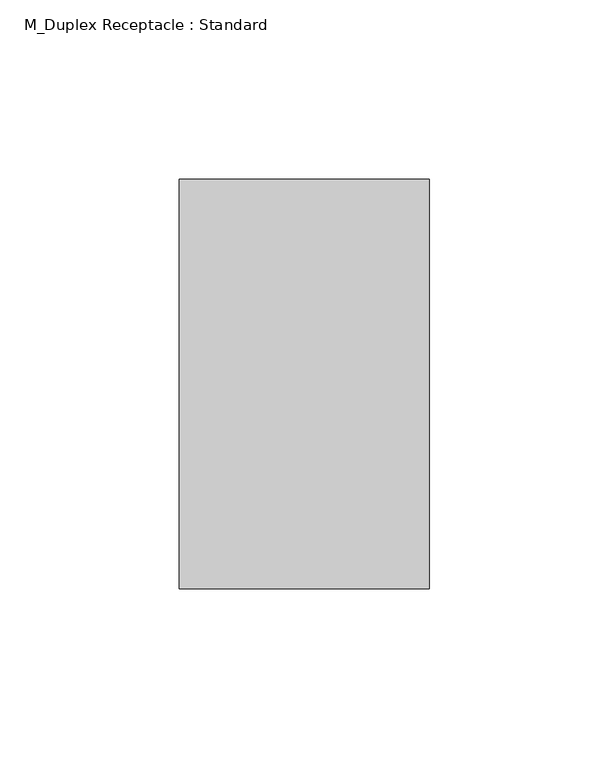
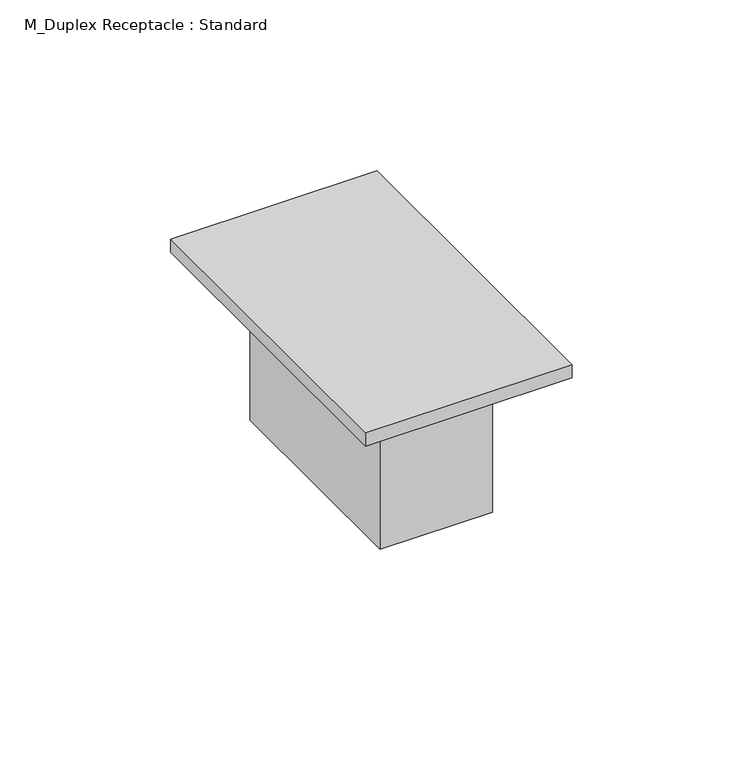
"""IFC4 building model written with IfcOpenShell, lengths in millimetres: proxy geometry, M_Duplex Receptacle : Standard."""

from ifc_helpers import new_model, si_unit, frame, origin, origin_with_axes, place, context, project, spatial, polyline, outline, extrude, source, transform, mapped, element, save


def m_duplex_receptacle_standard_10251bba(model_context):
    return source(origin(), model_context, "Body", "SweptSolid", [
        extrude(outline(polyline([(19.05, 38.1), (19.05, -38.1), (-19.05, -38.1), (-19.05, 38.1), (19.05, 38.1)])), frame((0.0, 0.0, -53.975), z_axis=(0.0, 0.0, 1.0), x_axis=(1.0, 0.0, 0.0)), (0.0, 0.0, 1.0), 53.975),
        extrude(outline(polyline([(34.925, 57.15), (34.925, -57.15), (-34.925, -57.15), (-34.925, 57.15), (34.925, 57.15)])), origin_with_axes(), (0.0, 0.0, 1.0), 4.7625),
    ])


if __name__ == "__main__":
    model = new_model("IFC4")
    model_context = context("Model", 3, world=origin())
    ifc_project = project(units=[si_unit("LENGTHUNIT", "METRE", prefix="MILLI")], contexts=[model_context])
    site = spatial("IfcSite", under=ifc_project)
    building = spatial("IfcBuilding", under=site)
    placement = place(None, origin())
    m_duplex_receptacle_standard_shape = m_duplex_receptacle_standard_10251bba(model_context)
    element("IfcBuildingElementProxy", 1, Name="M_Duplex Receptacle : Standard", ObjectType="M_Duplex Receptacle : Standard", at=placement, inside=building, context=model_context, shape_type="MappedRepresentation", body=[
        mapped(m_duplex_receptacle_standard_shape, transform((0.0, 0.0, 0.0), x_axis=(1.0, 0.0, 0.0), y_axis=(0.0, 1.0, 0.0), z_axis=(0.0, 0.0, 1.0))),
    ])
    save(model, "model.ifc")

# Revit data of these elements
# Type "M_Duplex Receptacle : Standard"
#   Label = ""
#   Switch Voltage = 120 V
#   Load = 180 VA
#   Default Elevation = 460 mm
#   Load Classification = Receptacle
#   Assembly Code = ""
